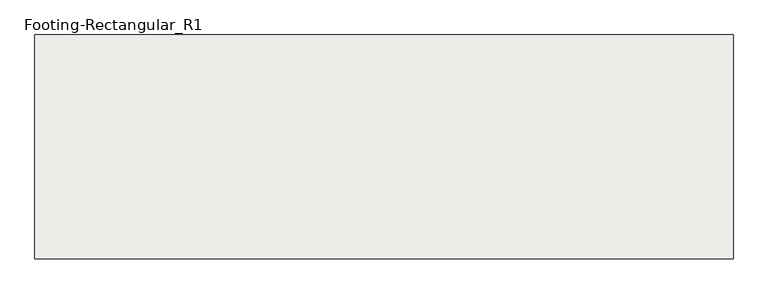
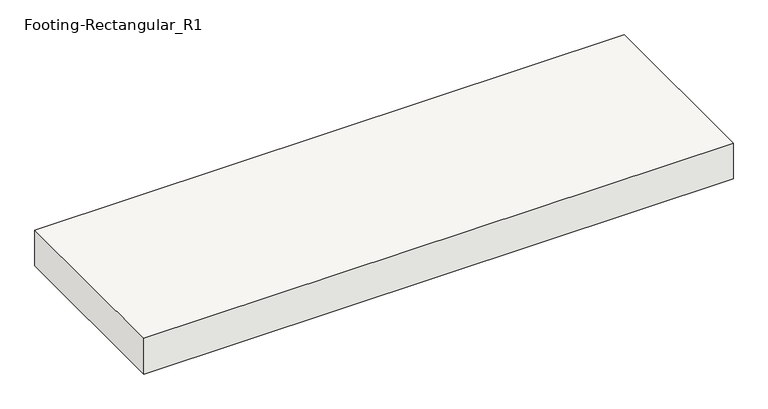
"""IFC4 building model written with IfcOpenShell, lengths in millimetres: slab geometry, Footing-Rectangular_R1 : H_SF_AR_S18_W7800xL2500xT500_Bitumen_F7."""

from ifc_helpers import new_model, si_unit, frame, origin, place, context, project, spatial, polyline, outline, extrude, source, transform, mapped, element, save


def footing_rectangular_r1_e1557040(model_context):
    return source(origin(), model_context, "Body", "SweptSolid", [
        extrude(outline(polyline([(3900.0, 1250.0), (3900.0, -1250.0), (-3900.0, -1250.0), (-3900.0, 1250.0), (3900.0, 1250.0)])), frame((0.0, 0.0, -500.0), z_axis=(0.0, 0.0, 1.0), x_axis=(1.0, 0.0, 0.0)), (0.0, 0.0, 1.0), 500.0),
    ])


if __name__ == "__main__":
    model = new_model("IFC4")
    model_context = context("Model", 3, world=origin())
    ifc_project = project(units=[si_unit("LENGTHUNIT", "METRE", prefix="MILLI")], contexts=[model_context])
    site = spatial("IfcSite", under=ifc_project)
    building = spatial("IfcBuilding", under=site)
    placement = place(None, origin())
    footing_rectangular_r1_shape = footing_rectangular_r1_e1557040(model_context)
    element("IfcSlab", 1, ObjectType="Footing-Rectangular_R1 : H_SF_AR_S18_W7800xL2500xT500_Bitumen_F7", at=placement, inside=building, context=model_context, shape_type="MappedRepresentation", body=[
        mapped(footing_rectangular_r1_shape, transform((0.0, 0.0, 0.0), x_axis=(1.0, 0.0, 0.0), y_axis=(0.0, 1.0, 0.0), z_axis=(0.0, 0.0, 1.0))),
    ])
    save(model, "model.ifc")

# Revit data of these elements
# Type "Footing-Rectangular_R1 : H_SF_AR_S18_W7800xL2500xT500_Bitumen_F7"
#   Type Mark = "F7"
#   Top bar = "D25@300"
#   Description = "UG Shallow Foundation"
#   Bottom bar = "D20@300"
#   Width = 7800 mm
#   Length = 2500 mm
#   Foundation Thickness = 500 mm
#   Structural Material [instance default] = none
#   Assembly Code = ""
